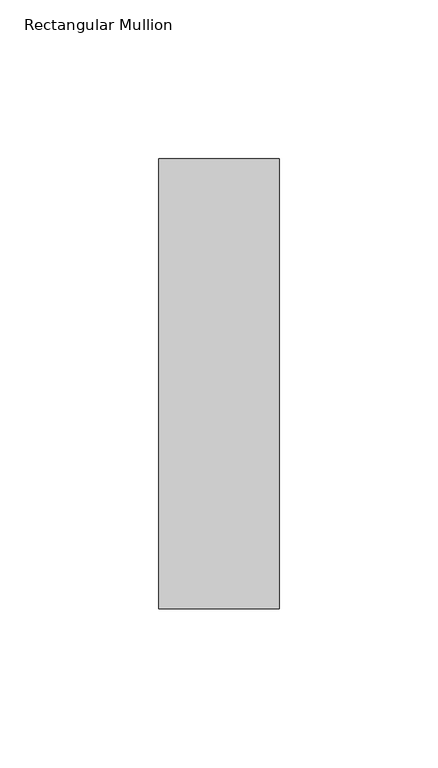
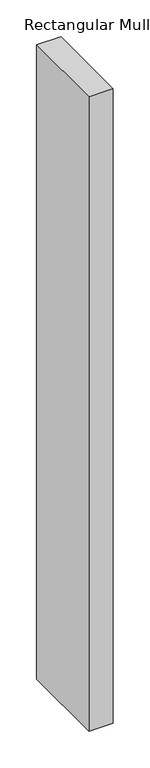
"""IFC4 building model written with IfcOpenShell, lengths in millimetres: member geometry, Rectangular Mullion : NLRS_21_CWM_hsb-regel 38x142_gen_rsf."""

from ifc_helpers import new_model, si_unit, frame, origin, place, context, project, spatial, polyline, outline, extrude, source, transform, mapped, element, save


def rectangular_mullion_a4b8200b(model_context):
    return source(origin(), model_context, "Body", "SweptSolid", [
        extrude(outline(polyline([(0.0, -71.0), (-38.0, -71.0), (-38.0, 71.0), (0.0, 71.0), (0.0, -71.0)])), frame((0.0, 0.0, -1050.0), z_axis=(0.0, 0.0, 1.0), x_axis=(1.0, 0.0, 0.0)), (0.0, 0.0, 1.0), 1050.0),
    ])


if __name__ == "__main__":
    model = new_model("IFC4")
    model_context = context("Model", 3, world=origin())
    ifc_project = project(units=[si_unit("LENGTHUNIT", "METRE", prefix="MILLI")], contexts=[model_context])
    site = spatial("IfcSite", under=ifc_project)
    building = spatial("IfcBuilding", under=site)
    placement = place(None, origin())
    rectangular_mullion_shape = rectangular_mullion_a4b8200b(model_context)
    element("IfcMember", 1, ObjectType="Rectangular Mullion : NLRS_21_CWM_hsb-regel 38x142_gen_rsf", at=placement, inside=building, context=model_context, shape_type="MappedRepresentation", body=[
        mapped(rectangular_mullion_shape, transform((0.0, 0.0, 0.0), x_axis=(1.0, 0.0, 0.0), y_axis=(0.0, 1.0, 0.0), z_axis=(0.0, 0.0, 1.0))),
    ])
    save(model, "model.ifc")

# Revit data of these elements
# Type "Rectangular Mullion : NLRS_21_CWM_hsb-regel 38x142_gen_rsf"
#   Export Type to IFC As = "IfcWall"
#   Type IfcGUID = "07M7mRoiH1CR8m_RSKIwpF"
#   Assembly Code = "21.10"
#   built-in parameter 1007322 = 0.465879 (stored number, unit not read)
#   built-in parameter 1007321 = 0.062336 (stored number, unit not read)
#   built-in parameter 1007320 = 0.062336 (stored number, unit not read)
# Element 1 (IfcMember, "Rectangular Mullion : NLRS_21_CWM_hsb-regel 38x142_gen_rsf")
#   Materials on its faces: "NLRS_i2_hout naaldhout vuren_gen_rsf"
# Materials
#   "NLRS_i2_hout naaldhout vuren_gen_rsf": class "I - Hout", colour RGB 234 199 147, transparency 0, Keynote = "i2", Manufacturer = "Revit Standards Foundation", URL = "www.revitstandards.org", Description = "hout vuren", Cost = 0
